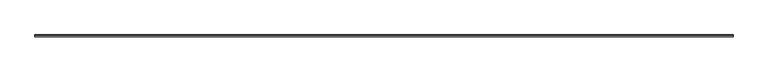
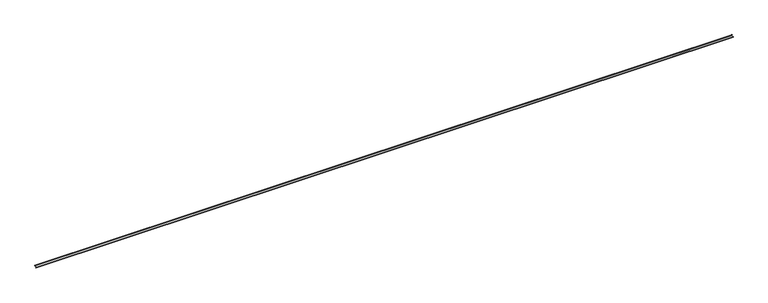
"""IFC4 building model written with IfcOpenShell, lengths in millimetres: proxy geometry, Generic Models 7:Generic Models 1:337419:Generic Models 1:337419 : Generic Models 7:Generic Models 1:337419:6 : Generic Models 7:Generic Models 1:337419:Generic Models 1:337419 : Generic Models 7:Generic Models 1:337419:301336."""

from ifc_helpers import new_model, si_unit, frame, origin, place, context, project, spatial, polyline, outline, extrude, source, transform, mapped, element, save


def generic_models_63425ecc(model_context):
    return source(origin(), model_context, "Body", "SweptSolid", [
        extrude(outline(polyline([(-567932.6413841, 6126.1625), (-568183.8632591, 6126.1625), (-568183.8632591, 6050.861086), (-568170.0763026, 6039.2924559), (-568172.0482374, 6037.320521), (-568186.6413841, 6049.565625), (-568186.6413841, 6128.940625), (-567935.4195091, 6128.940625), (-567935.4195091, 6210.592039), (-567949.0202751, 6222.0044367), (-567947.0483402, 6223.9763716), (-567932.6413841, 6211.8875), (-567932.6413841, 6126.1625)])), frame((578901.3117239, 0.0, 0.0), z_axis=(1.0, 0.0, 0.0), x_axis=(0.0, 1.0, 0.0)), (0.0, 0.0, 1.0), 88442.8),
    ])


if __name__ == "__main__":
    model = new_model("IFC4")
    model_context = context("Model", 3, world=origin())
    ifc_project = project(units=[si_unit("LENGTHUNIT", "METRE", prefix="MILLI")], contexts=[model_context])
    site = spatial("IfcSite", under=ifc_project)
    building = spatial("IfcBuilding", under=site)
    placement = place(None, origin())
    generic_models_shape = generic_models_63425ecc(model_context)
    element("IfcBuildingElementProxy", 1, Name="Generic Models 7:Generic Models 1:337419:Generic Models 1:337419 : Generic Models 7:Generic Models 1:337419:6 : Generic Models 7:Generic Models 1:337419:Generic Models 1:337419 : Generic Models 7:Generic Models 1:337419:301336", ObjectType="Generic Models 7:Generic Models 1:337419:Generic Models 1:337419 : Generic Models 7:Generic Models 1:337419:6 : Generic Models 7:Generic Models 1:337419:Generic Models 1:337419 : Generic Models 7:Generic Models 1:337419:301336", at=placement, inside=building, context=model_context, shape_type="MappedRepresentation", body=[
        mapped(generic_models_shape, transform((0.0, 0.0, 0.0), x_axis=(1.0, 0.0, 0.0), y_axis=(0.0, 1.0, 0.0), z_axis=(0.0, 0.0, 1.0))),
    ])
    save(model, "model.ifc")

# Revit data of these elements
# Type "Generic Models 7:Generic Models 1:337419:Generic Models 1:337419 : Generic Models 7:Generic Models 1:337419:6 : Generic Models 7:Generic Models 1:337419:Generic Models 1:337419 : Generic Models 7:Generic Models 1:337419:301336"
#   NameOverride = "Generic Models 7:Generic Models 1:337419:Generic Models 1:337419 : Generic Models 7:Generic Models 1:337419:301336"
#   ObjectTypeOverride = "Generic Models 1:337419 : Generic Models 7:Generic Models 1:337419"
#   Reference = "Generic Models 1"
#   Tag = "301336"
# Element 1 (IfcBuildingElementProxy, "Generic Models 7:Generic Models 1:337419:Generic Models 1:337419 : Generic Models 7:Generic Models 1:337419:6 : Generic Models 7:Generic Models 1:337419:Generic Models 1:337419 : Generic Models 7:Generic Models 1:337419:301336")
#   Materials on its faces: "'ZEE' SECTION (8.0x3.5Z - SEE STRUCT. DWGS)"
# Materials
#   "'ZEE' SECTION (8.0x3.5Z - SEE STRUCT. DWGS)": class "Unassigned", colour RGB 210 209 208, transparency 0, Keynote = "M05121300.02", Cost = 0
